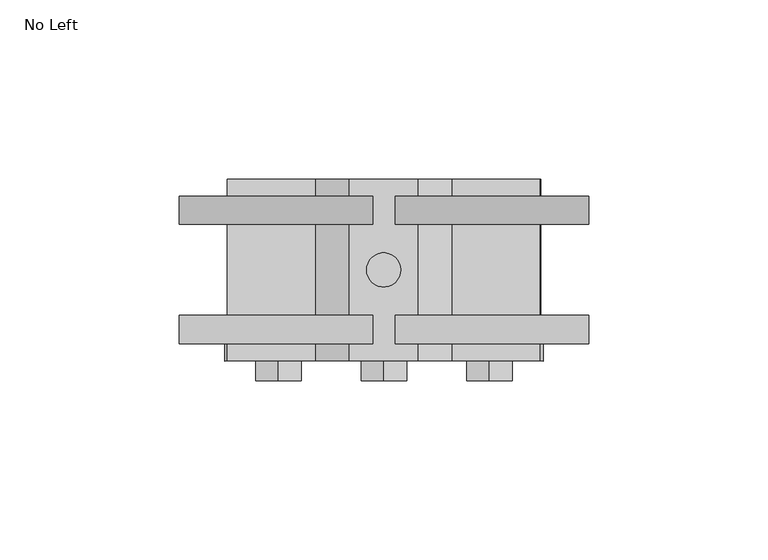
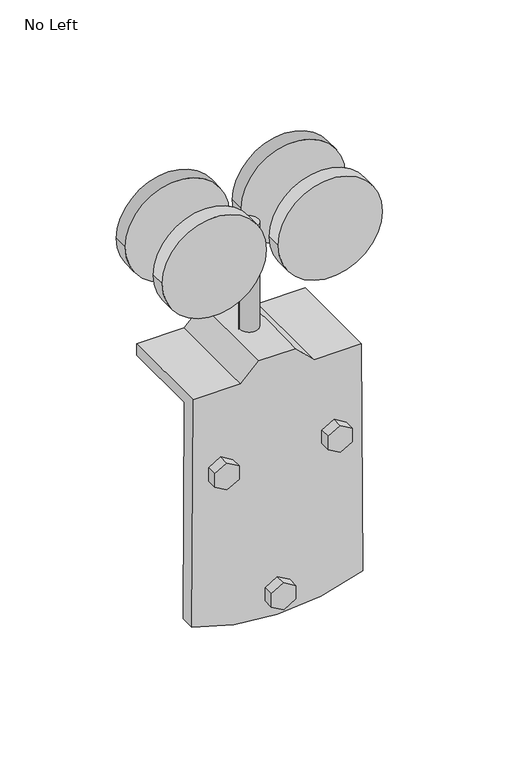
"""IFC4 building model written with IfcOpenShell, lengths in millimetres: proxy geometry, 087100_14 - Sliding and Folding Door Hardware - 5040 Box Rail Hangers : No Left."""

import ifcopenshell
import ifcopenshell.guid

model = None  # the IFC model being written
_history = None  # IfcOwnerHistory: only IFC2X3 demands one
_inside = {}  # id of a spatial element -> (the spatial element, [elements in it])
_under = {}  # id of a project, library or spatial element -> (it, [spatial elements below it])
_declared = {}  # id of a project -> (the project, [libraries it declares])
_typed = {}  # id of a type object -> (the type object, [elements of that type])
_made_of = {}  # id of a material, layer set ... -> (it, [elements and type objects made of it])


def new_model(schema):
    """Start an empty IFC model of exactly this schema.

    Asked for "IFC4X3", IfcOpenShell would pick the latest addendum, in which some entities
    have other attributes; the version numbers below select the first issue.
    IFC2X3 requires an IfcOwnerHistory on every rooted entity: one is made here for all.
    """
    global model, _history
    if schema == "IFC4X3":
        model = ifcopenshell.file(schema_version=(4, 3, 0, 0))
    else:
        model = ifcopenshell.file(schema=schema)
    _inside.clear()
    _under.clear()
    _declared.clear()
    _typed.clear()
    _made_of.clear()
    _history = None
    if model.schema == "IFC2X3":
        org = make("IfcOrganization", Name="unknown")
        user = make(
            "IfcPersonAndOrganization",
            ThePerson=make("IfcPerson", FamilyName="unknown"),
            TheOrganization=org,
        )
        app = make(
            "IfcApplication",
            ApplicationDeveloper=org,
            Version="unknown",
            ApplicationFullName="unknown",
            ApplicationIdentifier="unknown",
        )
        _history = make(
            "IfcOwnerHistory",
            OwningUser=user,
            OwningApplication=app,
            ChangeAction="ADDED",
            CreationDate=0,
        )
    return model


def make(cls, **values):
    """One entity of the class cls with the attributes given. An attribute that is None is left unset."""
    return model.create_entity(
        cls, **{name: value for name, value in values.items() if value is not None}
    )


def rooted(cls, **values):
    """An entity with a GlobalId (a new one), such as an element, a storey or a relation."""
    return make(cls, GlobalId=ifcopenshell.guid.new(), OwnerHistory=_history, **values)


def si_unit(unit_type, name, prefix=None):
    """IfcSIUnit, for example si_unit("LENGTHUNIT", "METRE", prefix="MILLI")."""
    return make("IfcSIUnit", UnitType=unit_type, Prefix=prefix, Name=name)


def assignment(units):
    """IfcUnitAssignment: the units of a project."""
    return None if units is None else make("IfcUnitAssignment", Units=units)


def point(xyz):
    """IfcCartesianPoint."""
    return None if xyz is None else make("IfcCartesianPoint", Coordinates=xyz)


def direction(xyz):
    """IfcDirection."""
    return None if xyz is None else make("IfcDirection", DirectionRatios=xyz)


def frame(location, z_axis=None, x_axis=None):
    """IfcAxis2Placement3D, a coordinate frame: its origin and axes. An axis left out is left unset."""
    return make(
        "IfcAxis2Placement3D",
        Location=point(location),
        Axis=direction(z_axis),
        RefDirection=direction(x_axis),
    )


def frame_2d(location, x_axis=None):
    """IfcAxis2Placement2D, a coordinate frame in the plane: its origin and x axis."""
    return make(
        "IfcAxis2Placement2D", Location=point(location), RefDirection=direction(x_axis)
    )


def origin():
    """The frame at (0, 0, 0) with its axes left unset."""
    return frame((0.0, 0.0, 0.0))


def origin_with_axes():
    """The frame at (0, 0, 0) with the z axis (0, 0, 1) and the x axis (1, 0, 0) written out."""
    return frame((0.0, 0.0, 0.0), z_axis=(0.0, 0.0, 1.0), x_axis=(1.0, 0.0, 0.0))


def place(relative_to, where):
    """IfcLocalPlacement: puts the frame where relative to a parent placement (None: the world)."""
    return make(
        "IfcLocalPlacement", PlacementRelTo=relative_to, RelativePlacement=where
    )


def context(
    kind, dimensions, precision=None, world=None, true_north=None, identifier=None
):
    """IfcGeometricRepresentationContext, for example the 3D "Model" context."""
    return make(
        "IfcGeometricRepresentationContext",
        ContextIdentifier=identifier,
        ContextType=kind,
        CoordinateSpaceDimension=dimensions,
        Precision=precision,
        WorldCoordinateSystem=world,
        TrueNorth=true_north,
    )


def project(units=None, contexts=None):
    """IfcProject with its units and contexts."""
    return rooted(
        "IfcProject",
        Name="project",
        RepresentationContexts=contexts,
        UnitsInContext=assignment(units),
    )


def spatial(cls, under=None, at=None, **own):
    """A site, building, storey or space (cls), placed at a placement, below another one or the project."""
    s = rooted(cls, ObjectPlacement=at, **own)
    if under is not None:
        _under.setdefault(under.id(), (under, []))[1].append(s)
    return s


def polyline(points):
    """IfcPolyline through the points."""
    return make("IfcPolyline", Points=[point(p) for p in points])


def circle_curve(where, radius):
    """IfcCircle in the frame where."""
    return make("IfcCircle", Position=where, Radius=radius)


def trimmed(basis, trim1, trim2, sense, master):
    """IfcTrimmedCurve: the piece of a basis curve between two trims."""
    return make(
        "IfcTrimmedCurve",
        BasisCurve=basis,
        Trim1=trim1,
        Trim2=trim2,
        SenseAgreement=sense,
        MasterRepresentation=master,
    )


def segment(curve, same_sense, transition):
    """IfcCompositeCurveSegment."""
    return make(
        "IfcCompositeCurveSegment",
        Transition=transition,
        SameSense=same_sense,
        ParentCurve=curve,
    )


def composite_curve(segments, self_intersect=None):
    """IfcCompositeCurve: segments joined end to end."""
    return make("IfcCompositeCurve", Segments=segments, SelfIntersect=self_intersect)


def outline(outer, holes=None, kind="AREA"):
    """IfcArbitraryClosedProfileDef: a profile drawn as a closed curve; with holes, ...WithVoids."""
    if holes is None:
        return make("IfcArbitraryClosedProfileDef", ProfileType=kind, OuterCurve=outer)
    return make(
        "IfcArbitraryProfileDefWithVoids",
        ProfileType=kind,
        OuterCurve=outer,
        InnerCurves=holes,
    )


def extrude(swept, where, along, depth):
    """IfcExtrudedAreaSolid: the profile swept, set in the frame where, extruded along a direction by depth."""
    return make(
        "IfcExtrudedAreaSolid",
        SweptArea=swept,
        Position=where,
        ExtrudedDirection=direction(along),
        Depth=depth,
    )


def shape(context_of_items, identifier, shape_type, items):
    """IfcShapeRepresentation: the items that make up one representation, for example the "Body"."""
    return make(
        "IfcShapeRepresentation",
        ContextOfItems=context_of_items,
        RepresentationIdentifier=identifier,
        RepresentationType=shape_type,
        Items=items,
    )


def source(mapping_origin, context_of_items, identifier, shape_type, items):
    """IfcRepresentationMap: a shape defined once, which mapped items show again and again."""
    return make(
        "IfcRepresentationMap",
        MappingOrigin=mapping_origin,
        MappedRepresentation=shape(context_of_items, identifier, shape_type, items),
    )


def transform(
    local_origin,
    x_axis=None,
    y_axis=None,
    z_axis=None,
    scale=None,
    scale2=None,
    scale3=None,
    uniform=True,
):
    """IfcCartesianTransformationOperator3D, or its non-uniform kind. x_axis, y_axis, z_axis: its Axis1, 2, 3."""
    if uniform:
        return make(
            "IfcCartesianTransformationOperator3D",
            Axis1=direction(x_axis),
            Axis2=direction(y_axis),
            LocalOrigin=point(local_origin),
            Scale=scale,
            Axis3=direction(z_axis),
        )
    return make(
        "IfcCartesianTransformationOperator3DnonUniform",
        Axis1=direction(x_axis),
        Axis2=direction(y_axis),
        LocalOrigin=point(local_origin),
        Scale=scale,
        Axis3=direction(z_axis),
        Scale2=scale2,
        Scale3=scale3,
    )


def mapped(mapping_source, mapping_target):
    """IfcMappedItem: shows the shape of a source again, moved by a transform."""
    return make(
        "IfcMappedItem", MappingSource=mapping_source, MappingTarget=mapping_target
    )


def made_of(thing, what):
    """Note that an element or type object is made of a material, layer set ...; save() writes the relation."""
    if what is not None:
        _made_of.setdefault(what.id(), (what, []))[1].append(thing)
    return thing


def element(
    cls,
    number,
    at=None,
    inside=None,
    cuts=None,
    type_object=None,
    material=None,
    context=None,
    identifier="Body",
    shape_type=None,
    held_by="IfcProductDefinitionShape",
    body=None,
    shapes=None,
    **own,
):
    """One element of the class cls, such as IfcWall. Its Tag is "e" and its number.

    at: its placement. inside: the storey or other place that contains it. cuts: it is an
    opening in that element (IfcRelVoidsElement). A single representation is given by context,
    identifier, shape_type and body (its items); several are given by shapes. held_by: the class
    of the entity that holds the representations. save() writes the other relations.
    """
    e = rooted(cls, Tag="e%d" % number, ObjectPlacement=at, **own)
    if body is not None:
        shapes = [shape(context, identifier, shape_type, body)]
    if shapes is not None:
        e.Representation = make(held_by, Representations=shapes)
    if inside is not None:
        _inside.setdefault(inside.id(), (inside, []))[1].append(e)
    if cuts is not None:
        rooted(
            "IfcRelVoidsElement", RelatingBuildingElement=cuts, RelatedOpeningElement=e
        )
    if type_object is not None:
        _typed.setdefault(type_object.id(), (type_object, []))[1].append(e)
    return made_of(e, material)


def aggregate(whole, parts):
    """IfcRelAggregates: a whole, such as a stair, and the parts it consists of."""
    return rooted("IfcRelAggregates", RelatingObject=whole, RelatedObjects=parts)


def save(model, path):
    """Write the relations noted so far, then the file.

    IfcRelAggregates (storeys below a building ...), IfcRelContainedInSpatialStructure (elements
    in a storey), IfcRelDefinesByType, IfcRelAssociatesMaterial and IfcRelDeclares: one each for
    every whole, place, type object, material and project.
    """
    for whole, parts in _under.values():
        aggregate(whole, parts)
    for where, things in _inside.values():
        rooted(
            "IfcRelContainedInSpatialStructure",
            RelatedElements=things,
            RelatingStructure=where,
        )
    for kind, things in _typed.values():
        rooted("IfcRelDefinesByType", RelatedObjects=things, RelatingType=kind)
    for what, things in _made_of.values():
        rooted("IfcRelAssociatesMaterial", RelatedObjects=things, RelatingMaterial=what)
    for by, libraries in _declared.values():
        rooted("IfcRelDeclares", RelatingContext=by, RelatedDefinitions=libraries)
    model.write(path)


def plane_surface(at):
    """IfcPlane: the flat surface through the origin of the frame at, square to its z axis."""
    return make("IfcPlane", Position=at)


def cylinder_surface(at, radius):
    """IfcCylindricalSurface: all points at the distance radius from the z axis of the frame at."""
    return make("IfcCylindricalSurface", Position=at, Radius=radius)


def advanced_brep(points, edges, surfaces, faces):
    """IfcAdvancedBrep: a solid bounded by faces that lie on surfaces and meet in shared edges.

    An edge is (start, end): straight between two places in points (the first is 0);
    or (start, end, curve); or (start, end, curve, False) where it runs against its curve.
    A face is (place in surfaces, loops), or (place, loops, False) where it looks against
    its surface's normal. A loop lists edges by number (the first is 1), with a minus sign
    where the edge is run from its end to its start. The first loop is the outer one.
    """
    corners = [point(p) for p in points]
    vertices = [make("IfcVertexPoint", VertexGeometry=c) for c in corners]
    made = []
    for start, end, *more in edges:
        made.append(
            make(
                "IfcEdgeCurve",
                EdgeStart=vertices[start],
                EdgeEnd=vertices[end],
                EdgeGeometry=more[0] if more else make("IfcPolyline", Points=[corners[start], corners[end]]),
                SameSense=more[1] if len(more) > 1 else True,
            )
        )
    hull = []
    for where, loops, *sense in faces:
        bounds = []
        for j, loop in enumerate(loops):
            ring = [make("IfcOrientedEdge", EdgeElement=made[abs(k) - 1], Orientation=k > 0) for k in loop]
            bounds.append(
                make(
                    "IfcFaceOuterBound" if j == 0 else "IfcFaceBound",
                    Bound=make("IfcEdgeLoop", EdgeList=ring),
                    Orientation=True,
                )
            )
        hull.append(make("IfcAdvancedFace", Bounds=bounds, FaceSurface=surfaces[where], SameSense=sense[0] if sense else True))
    return make("IfcAdvancedBrep", Outer=make("IfcClosedShell", CfsFaces=hull))


def no_left_8841d9be(model_context):
    return source(origin(), model_context, "Body", "SolidModel", [
        extrude(outline(polyline([(-117.3880521, -6.35), (-121.0542263, 0.0), (-117.3880521, 6.35), (-110.0557037, 6.35), (-106.3895295, 0.0), (-110.0557037, -6.35), (-117.3880521, -6.35)])), frame((0.0, 9.525, 0.0), z_axis=(0.0, 1.0, 0.0), x_axis=(0.0, 0.0, 1.0)), (0.0, 0.0, 1.0), 5.55625),
        extrude(outline(polyline([(-110.0557037, -6.35), (-117.3880521, -6.35), (-121.0542263, 0.0), (-117.3880521, 6.35), (-110.0557037, 6.35), (-106.3895295, 0.0), (-110.0557037, -6.35)])), frame((0.0, -30.95625, 0.0), z_axis=(0.0, 1.0, 0.0), x_axis=(0.0, 0.0, 1.0)), (0.0, 0.0, 1.0), 5.55625),
        extrude(outline(composite_curve([segment(trimmed(circle_curve(frame_2d((-113.7218779, 0.0)), 3.96875), [point((-113.7218779, -3.96875))], [point((-113.7218779, 3.96875))], False, "CARTESIAN"), True, "CONTINUOUS"), segment(trimmed(circle_curve(frame_2d((-113.7218779, 0.0)), 3.96875), [point((-113.7218779, 3.96875))], [point((-113.7218779, -3.96875))], False, "CARTESIAN"), True, "CONTINUOUS")], self_intersect=False)), frame((0.0, -25.4, 0.0), z_axis=(0.0, 1.0, 0.0), x_axis=(0.0, 0.0, 1.0)), (0.0, 0.0, 1.0), 44.45),
        extrude(outline(polyline([(-33.8196076, -35.8279106), (-41.151956, -35.8279106), (-44.8181303, -29.4779106), (-41.151956, -23.1279106), (-33.8196076, -23.1279106), (-30.1534334, -29.4779106), (-33.8196076, -35.8279106)])), frame((0.0, -30.95625, 0.0), z_axis=(0.0, 1.0, 0.0), x_axis=(0.0, 0.0, 1.0)), (0.0, 0.0, 1.0), 5.55625),
        extrude(outline(composite_curve([segment(trimmed(circle_curve(frame_2d((-37.4857818, -29.4779106)), 3.96875), [point((-37.4857818, -33.4466606))], [point((-37.4857818, -25.5091606))], False, "CARTESIAN"), True, "CONTINUOUS"), segment(trimmed(circle_curve(frame_2d((-37.4857818, -29.4779106)), 3.96875), [point((-37.4857818, -25.5091606))], [point((-37.4857818, -33.4466606))], False, "CARTESIAN"), True, "CONTINUOUS")], self_intersect=False)), frame((0.0, -25.4, 0.0), z_axis=(0.0, 1.0, 0.0), x_axis=(0.0, 0.0, 1.0)), (0.0, 0.0, 1.0), 25.4),
        extrude(outline(polyline([(-41.151956, 23.1279765), (-44.8181303, 29.4779765), (-41.151956, 35.8279765), (-33.8196076, 35.8279765), (-30.1534334, 29.4779765), (-33.8196076, 23.1279765), (-41.151956, 23.1279765)])), frame((0.0, 9.525, 0.0), z_axis=(0.0, 1.0, 0.0), x_axis=(0.0, 0.0, 1.0)), (0.0, 0.0, 1.0), 5.55625),
        extrude(outline(polyline([(-33.8196076, 23.1279765), (-41.151956, 23.1279765), (-44.8181303, 29.4779765), (-41.151956, 35.8279765), (-33.8196076, 35.8279765), (-30.1534334, 29.4779765), (-33.8196076, 23.1279765)])), frame((0.0, -30.95625, 0.0), z_axis=(0.0, 1.0, 0.0), x_axis=(0.0, 0.0, 1.0)), (0.0, 0.0, 1.0), 5.55625),
        extrude(outline(composite_curve([segment(trimmed(circle_curve(frame_2d((-37.4857818, 29.4779765)), 3.96875), [point((-37.4857818, 25.5092265))], [point((-37.4857818, 33.4467265))], False, "CARTESIAN"), True, "CONTINUOUS"), segment(trimmed(circle_curve(frame_2d((-37.4857818, 29.4779765)), 3.96875), [point((-37.4857818, 33.4467265))], [point((-37.4857818, 25.5092265))], False, "CARTESIAN"), True, "CONTINUOUS")], self_intersect=False)), frame((0.0, -25.4, 0.0), z_axis=(0.0, 1.0, 0.0), x_axis=(0.0, 0.0, 1.0)), (0.0, 0.0, 1.0), 44.45),
        advanced_brep(
        [(-44.4707374, -25.4, -118.5726247), (44.4707374, -25.4, -118.5726247), (43.7118564, -25.4, 6.35), (19.0589621, -25.4, 6.35), (9.6563712, -25.4, 15.7523786), (-9.6566784, -25.4, 15.7523786), (-19.059057, -25.4, 6.35), (-43.7119983, -25.4, 6.35), (-25.119743, -25.4, -33.1275483), (-25.119743, -25.4, -41.8440154), (-33.8360782, -25.4, -41.8440154), (-33.8360782, -25.4, -33.1275483), (33.8360782, -25.4, -33.1275483), (33.8360782, -25.4, -41.8440154), (25.1198748, -25.4, -41.8440154), (25.1198748, -25.4, -33.1275483), (4.3581017, -25.4, -109.3636444), (4.3581017, -25.4, -118.0801114), (-4.3581017, -25.4, -118.0801114), (-4.3581017, -25.4, -109.3636444), (-43.7119983, 25.4, 6.35), (-19.059057, 25.4, 6.35), (-9.6566784, 25.4, 15.7523786), (9.6563712, 25.4, 15.7523786), (19.0589621, 25.4, 6.35), (43.7118564, 25.4, 6.35), (43.7504315, 25.4, 0.0), (16.428748, 25.4, 0.0), (7.0261571, 25.4, 9.4023786), (-7.0264223, 25.4, 9.4023786), (-16.4288009, 25.4, 0.0), (-43.7505662, 25.4, 0.0), (-43.7505662, -17.4625, 0.0), (-44.4707374, -17.4625, -118.5726247), (-16.4288009, -17.4625, 0.0), (-7.0264223, -17.4625, 9.4023786), (7.0261571, -17.4625, 9.4023786), (16.428748, -17.4625, 0.0), (43.7504315, -17.4625, 0.0), (44.4707374, -17.4625, -118.5726247), (19.0589621, -17.4625, 6.35), (9.6563712, -17.4625, 15.7523786), (-9.6566784, -17.4625, 15.7523786), (-19.059057, -17.4625, 6.35), (-25.119743, -17.4625, -33.1275483), (-33.8360782, -17.4625, -33.1275483), (-33.8360782, -17.4625, -41.8440154), (-25.119743, -17.4625, -41.8440154), (33.8360782, -17.4625, -33.1275483), (25.1198748, -17.4625, -33.1275483), (25.1198748, -17.4625, -41.8440154), (33.8360782, -17.4625, -41.8440154), (4.3581017, -17.4625, -109.3636444), (-4.3581017, -17.4625, -109.3636444), (-4.3581017, -17.4625, -118.0801114), (4.3581017, -17.4625, -118.0801114)],
        [
            (0, 1, circle_curve(frame((0.0, -25.4, -6.3557626), z_axis=(0.0, -1.0, 0.0), x_axis=(1.0, 0.0, 0.0)), 120.7073761)),
            (1, 2),
            (2, 3),
            (3, 4),
            (4, 5),
            (5, 6),
            (6, 7),
            (7, 0),
            (8, 9),
            (9, 10),
            (10, 11),
            (11, 8),
            (12, 13),
            (13, 14),
            (14, 15),
            (15, 12),
            (16, 17),
            (17, 18),
            (18, 19),
            (19, 16),
            (20, 21),
            (21, 22),
            (22, 23),
            (23, 24),
            (24, 25),
            (25, 26),
            (26, 27),
            (27, 28),
            (28, 29),
            (29, 30),
            (30, 31),
            (31, 20),
            (7, 20),
            (31, 32),
            (32, 33),
            (33, 0),
            (30, 34),
            (34, 32),
            (29, 35),
            (35, 34),
            (28, 36),
            (36, 35),
            (27, 37),
            (37, 36),
            (26, 38),
            (38, 37),
            (1, 39),
            (39, 38),
            (25, 2),
            (24, 40),
            (40, 3),
            (23, 41),
            (41, 4),
            (22, 42),
            (42, 5),
            (21, 43),
            (43, 6),
            (39, 33, circle_curve(frame((0.0, -17.4625, -6.3557626), z_axis=(0.0, 1.0, 0.0), x_axis=(1.0, 0.0, 0.0)), 120.7073761)),
            (44, 45),
            (45, 46),
            (46, 47),
            (47, 44),
            (48, 49),
            (49, 50),
            (50, 51),
            (51, 48),
            (52, 53),
            (53, 54),
            (54, 55),
            (55, 52),
            (8, 44),
            (47, 9),
            (46, 10),
            (45, 11),
            (12, 48),
            (51, 13),
            (50, 14),
            (49, 15),
            (16, 52),
            (55, 17),
            (54, 18),
            (53, 19),
        ],
        [
            plane_surface(frame((-46.969086, -25.4, -529.9133004), z_axis=(0.0, -1.0, 0.0), x_axis=(-0.006073560512695754, 0.0, -0.9999815557612544))),
            plane_surface(frame((-46.969086, 25.4, -529.9133004), z_axis=(0.0, 1.0, 0.0), x_axis=(0.006073560512695754, 0.0, 0.9999815557612544))),
            plane_surface(frame((-43.7119983, -25.4, 6.35), z_axis=(-0.9999815557612544, 0.0, 0.006073560512695754), x_axis=(0.0, 1.0, 0.0))),
            plane_surface(frame((-43.7505662, -25.4, 0.0), z_axis=(0.0, 0.0, -1.0), x_axis=(0.0, 1.0, 0.0))),
            plane_surface(frame((-16.4288009, -25.4, 0.0), z_axis=(0.7071067811865476, 0.0, -0.7071067811865476), x_axis=(0.0, 1.0, 0.0))),
            plane_surface(frame((-7.0264223, -25.4, 9.4023786), z_axis=(0.0, 0.0, -1.0), x_axis=(0.0, 1.0, 0.0))),
            plane_surface(frame((7.0261571, -25.4, 9.4023786), z_axis=(-0.7070987963768838, 0.0, -0.7071147659060459), x_axis=(0.0, 1.0, 0.0))),
            plane_surface(frame((16.428748, -25.4, 0.0), z_axis=(0.0, 0.0, -1.0), x_axis=(0.0, 1.0, 0.0))),
            plane_surface(frame((43.7504315, -25.4, 0.0), z_axis=(0.9999815488618892, 0.0, 0.006074696352680505), x_axis=(0.0, 1.0, 0.0))),
            plane_surface(frame((43.7118564, -25.4, 6.35), z_axis=(0.0, 0.0, 1.0), x_axis=(0.0, 1.0, 0.0))),
            plane_surface(frame((19.0589621, -25.4, 6.35), z_axis=(0.7070987963768809, 0.0, 0.7071147659060488), x_axis=(0.0, 1.0, 0.0))),
            plane_surface(frame((9.6563712, -25.4, 15.7523786), z_axis=(0.0, 0.0, 1.0), x_axis=(0.0, 1.0, 0.0))),
            plane_surface(frame((-9.6566784, -25.4, 15.7523786), z_axis=(-0.7071067811865457, 0.0, 0.7071067811865495), x_axis=(0.0, 1.0, 0.0))),
            plane_surface(frame((-19.059057, -25.4, 6.35), z_axis=(0.0, 0.0, 1.0), x_axis=(0.0, 1.0, 0.0))),
            plane_surface(frame((-46.969086, -17.4625, -529.9133004), z_axis=(0.0, 1.0, 0.0), x_axis=(0.006073560512693812, 0.0, 0.9999815557612544))),
            cylinder_surface(frame((0.0, -17.4625, -6.3557626), z_axis=(0.0, -1.0, 0.0), x_axis=(1.0, 0.0, 0.0)), 120.7073761),
            plane_surface(frame((-25.119743, -25.4, -33.1275483), z_axis=(-1.0, 0.0, 0.0), x_axis=(0.0, 1.0, 0.0))),
            plane_surface(frame((-25.119743, -25.4, -41.8440154), z_axis=(0.0, 0.0, 1.0), x_axis=(0.0, 1.0, 0.0))),
            plane_surface(frame((-33.8360782, -25.4, -41.8440154), z_axis=(1.0, 0.0, 0.0), x_axis=(0.0, 1.0, 0.0))),
            plane_surface(frame((-33.8360782, -25.4, -33.1275483), z_axis=(0.0, 0.0, -1.0), x_axis=(0.0, 1.0, 0.0))),
            plane_surface(frame((33.8360782, -25.4, -33.1275483), z_axis=(-1.0, 0.0, 0.0), x_axis=(0.0, 1.0, 0.0))),
            plane_surface(frame((33.8360782, -25.4, -41.8440154), z_axis=(0.0, 0.0, 1.0), x_axis=(0.0, 1.0, 0.0))),
            plane_surface(frame((25.1198748, -25.4, -41.8440154), z_axis=(1.0, 0.0, 0.0), x_axis=(0.0, 1.0, 0.0))),
            plane_surface(frame((25.1198748, -25.4, -33.1275483), z_axis=(0.0, 0.0, -1.0), x_axis=(0.0, 1.0, 0.0))),
            plane_surface(frame((4.3581017, -25.4, -109.3636444), z_axis=(-1.0, 0.0, 0.0), x_axis=(0.0, 1.0, 0.0))),
            plane_surface(frame((4.3581017, -25.4, -118.0801114), z_axis=(0.0, 0.0, 1.0), x_axis=(0.0, 1.0, 0.0))),
            plane_surface(frame((-4.3581017, -25.4, -118.0801114), z_axis=(1.0, 0.0, 0.0), x_axis=(0.0, 1.0, 0.0))),
            plane_surface(frame((-4.3581017, -25.4, -109.3636444), z_axis=(0.0, 0.0, -1.0), x_axis=(0.0, 1.0, 0.0))),
        ],
        [
            (0, [[1, 2, 3, 4, 5, 6, 7, 8], [9, 10, 11, 12], [13, 14, 15, 16], [17, 18, 19, 20]]),
            (1, [[21, 22, 23, 24, 25, 26, 27, 28, 29, 30, 31, 32]]),
            (2, [[-8, 33, -32, 34, 35, 36]]),
            (3, [[-31, 37, 38, -34]]),
            (4, [[-30, 39, 40, -37]]),
            (5, [[-29, 41, 42, -39]]),
            (6, [[-28, 43, 44, -41]]),
            (7, [[-27, 45, 46, -43]]),
            (8, [[-2, 47, 48, -45, -26, 49]]),
            (9, [[-3, -49, -25, 50, 51]]),
            (10, [[-4, -51, -50, -24, 52, 53]]),
            (11, [[-5, -53, -52, -23, 54, 55]]),
            (12, [[-6, -55, -54, -22, 56, 57]]),
            (13, [[-33, -7, -57, -56, -21]]),
            (14, [[58, -35, -38, -40, -42, -44, -46, -48], [59, 60, 61, 62], [63, 64, 65, 66], [67, 68, 69, 70]]),
            (15, [[-1, -36, -58, -47]]),
            (16, [[-9, 71, -62, 72]]),
            (17, [[-10, -72, -61, 73]]),
            (18, [[-11, -73, -60, 74]]),
            (19, [[-12, -74, -59, -71]]),
            (20, [[-13, 75, -66, 76]]),
            (21, [[-14, -76, -65, 77]]),
            (22, [[-15, -77, -64, 78]]),
            (23, [[-16, -78, -63, -75]]),
            (24, [[-17, 79, -70, 80]]),
            (25, [[-18, -80, -69, 81]]),
            (26, [[-19, -81, -68, 82]]),
            (27, [[-20, -82, -67, -79]]),
        ],
    ),
        extrude(outline(composite_curve([segment(trimmed(circle_curve(frame_2d((71.8251107, -30.1481535)), 27.0838855), [point((71.8251107, -57.232039))], [point((71.8251107, -3.0642681))], False, "CARTESIAN"), True, "CONTINUOUS"), segment(trimmed(circle_curve(frame_2d((71.8251107, -30.1481535)), 27.0838855), [point((71.8251107, -3.0642681))], [point((71.8251107, -57.232039))], False, "CARTESIAN"), True, "CONTINUOUS")], self_intersect=False)), frame((0.0, 12.7, 0.0), z_axis=(0.0, 1.0, 0.0), x_axis=(0.0, 0.0, 1.0)), (0.0, 0.0, 1.0), 7.9375),
        extrude(outline(composite_curve([segment(trimmed(circle_curve(frame_2d((71.8251107, 30.2054611)), 27.0838855), [point((71.8251107, 3.1215756))], [point((71.8251107, 57.2893465))], False, "CARTESIAN"), True, "CONTINUOUS"), segment(trimmed(circle_curve(frame_2d((71.8251107, 30.2054611)), 27.0838855), [point((71.8251107, 57.2893465))], [point((71.8251107, 3.1215756))], False, "CARTESIAN"), True, "CONTINUOUS")], self_intersect=False)), frame((0.0, 12.7, 0.0), z_axis=(0.0, 1.0, 0.0), x_axis=(0.0, 0.0, 1.0)), (0.0, 0.0, 1.0), 7.9375),
        extrude(outline(composite_curve([segment(trimmed(circle_curve(frame_2d((-0.0657734, 0.0)), 4.7625), [point((-4.8282734, 0.0))], [point((4.6967266, 0.0))], False, "CARTESIAN"), True, "CONTINUOUS"), segment(trimmed(circle_curve(frame_2d((-0.0657734, 0.0)), 4.7625), [point((4.6967266, 0.0))], [point((-4.8282734, 0.0))], False, "CARTESIAN"), True, "CONTINUOUS")], self_intersect=False)), origin_with_axes(), (0.0, 0.0, 1.0), 73.5534737),
        extrude(outline(composite_curve([segment(trimmed(circle_curve(frame_2d((71.8251107, -30.1481535)), 27.0838855), [point((71.8251107, -57.232039))], [point((71.8251107, -3.0642681))], False, "CARTESIAN"), True, "CONTINUOUS"), segment(trimmed(circle_curve(frame_2d((71.8251107, -30.1481535)), 27.0838855), [point((71.8251107, -3.0642681))], [point((71.8251107, -57.232039))], False, "CARTESIAN"), True, "CONTINUOUS")], self_intersect=False)), frame((0.0, -20.6375, 0.0), z_axis=(0.0, 1.0, 0.0), x_axis=(0.0, 0.0, 1.0)), (0.0, 0.0, 1.0), 7.9375),
        extrude(outline(composite_curve([segment(trimmed(circle_curve(frame_2d((71.8251107, 30.2054611)), 27.0838855), [point((71.8251107, 3.1215756))], [point((71.8251107, 57.2893465))], False, "CARTESIAN"), True, "CONTINUOUS"), segment(trimmed(circle_curve(frame_2d((71.8251107, 30.2054611)), 27.0838855), [point((71.8251107, 57.2893465))], [point((71.8251107, 3.1215756))], False, "CARTESIAN"), True, "CONTINUOUS")], self_intersect=False)), frame((0.0, -20.6375, 0.0), z_axis=(0.0, 1.0, 0.0), x_axis=(0.0, 0.0, 1.0)), (0.0, 0.0, 1.0), 7.9375),
    ])


if __name__ == "__main__":
    model = new_model("IFC4")
    model_context = context("Model", 3, world=origin())
    ifc_project = project(units=[si_unit("LENGTHUNIT", "METRE", prefix="MILLI")], contexts=[model_context])
    site = spatial("IfcSite", under=ifc_project)
    building = spatial("IfcBuilding", under=site)
    placement = place(None, origin())
    no_left_shape = no_left_8841d9be(model_context)
    element("IfcBuildingElementProxy", 1, Name="087100_14 - Sliding and Folding Door Hardware - 5040 Box Rail Hangers : No Left", ObjectType="087100_14 - Sliding and Folding Door Hardware - 5040 Box Rail Hangers : No Left", at=placement, inside=building, context=model_context, shape_type="MappedRepresentation", body=[
        mapped(no_left_shape, transform((0.0, 0.0, 0.0), x_axis=(1.0, 0.0, 0.0), y_axis=(0.0, 1.0, 0.0), z_axis=(0.0, 0.0, 1.0))),
    ])
    save(model, "model.ifc")

# Revit data of these elements
# Type "087100_14 - Sliding and Folding Door Hardware - 5040 Box Rail Hangers : No Left"
#   Default Elevation = 4' - 0"
#   Left Bolt = element 2408421
#   Bracket Material = BOX RAIL HANGER W/ GALV. FASTNERS (NATIONAL 5040)
#   Bottom Bolt = element 2408420
# Element 1 (IfcBuildingElementProxy, "087100_14 - Sliding and Folding Door Hardware - 5040 Box Rail Hangers : No Left")
#   Materials on its faces: "STRUCTURAL BOLTS (PAINT TO MATCH STEEL FINISH)", "BOX RAIL HANGER W/ GALV. FASTNERS (NATIONAL 5040)"
# Materials
#   "BOX RAIL HANGER W/ GALV. FASTNERS (NATIONAL 5040)": class "Metal", colour RGB 199 199 199, transparency 0, Description = "Structural steel, ASTM A36 Grade B, mill finish", Cost = 0
#   "STRUCTURAL BOLTS (PAINT TO MATCH STEEL FINISH)": class "Generic", colour RGB 120 120 120, transparency 0, Cost = 0
